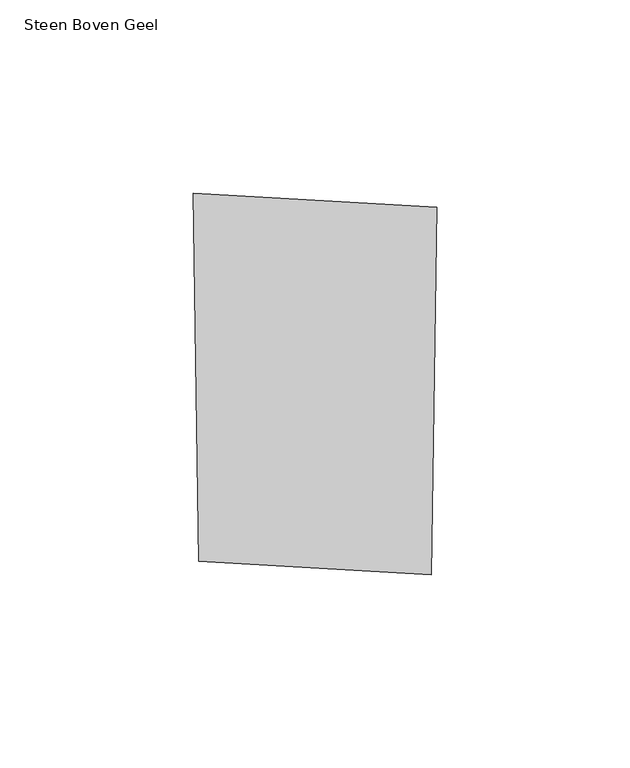
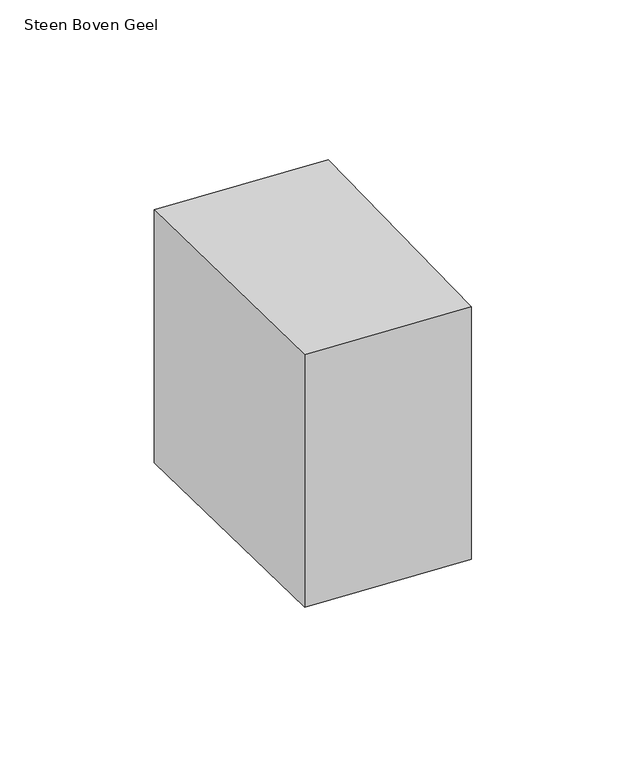
"""IFC4 building model written with IfcOpenShell, lengths in millimetres: proxy geometry, 00_GMA_steen_versie_4 : Steen Boven Geel."""

from ifc_helpers import new_model, si_unit, origin, origin_with_axes, place, context, project, spatial, polyline, outline, extrude, source, transform, mapped, element, save


def steen_boven_geel_85e85a47(model_context):
    return source(origin(), model_context, "Body", "SweptSolid", [
        extrude(outline(polyline([(101.271578, 118.9291664), (99.9224019, 23.8420556), (39.7241554, 27.3305171), (38.3007414, 122.5859361), (101.271578, 118.9291664)])), origin_with_axes(), (0.0, 0.0, 1.0), 100.0),
    ])


if __name__ == "__main__":
    model = new_model("IFC4")
    model_context = context("Model", 3, world=origin())
    ifc_project = project(units=[si_unit("LENGTHUNIT", "METRE", prefix="MILLI")], contexts=[model_context])
    site = spatial("IfcSite", under=ifc_project)
    building = spatial("IfcBuilding", under=site)
    placement = place(None, origin())
    steen_boven_geel_shape = steen_boven_geel_85e85a47(model_context)
    element("IfcBuildingElementProxy", 1, Name="00_GMA_steen_versie_4 : Steen Boven Geel", ObjectType="00_GMA_steen_versie_4 : Steen Boven Geel", at=placement, inside=building, context=model_context, shape_type="MappedRepresentation", body=[
        mapped(steen_boven_geel_shape, transform((0.0, 0.0, 0.0), x_axis=(1.0, 0.0, 0.0), y_axis=(0.0, 1.0, 0.0), z_axis=(0.0, 0.0, 1.0))),
    ])
    save(model, "model.ifc")

# Revit data of these elements
# Type "00_GMA_steen_versie_4 : Steen Boven Geel"
#   StootVoegHalfBoven [instance default] = 5 mm
#   StootVoegHalf [instance default] = 5 mm
#   StootVoegBreedteOnder = 10 mm
#   StootVoegBreedteBoven = 10 mm
#   Steendikte = 100 mm
#   LintVoegOnderHalf = 5 mm
#   LintVoegOnder = 10 mm
#   LintVoegBovenHalf = 0 mm
#   LintVoegBoven = 0 mm
#   materiaal = 21_steen_geel
#   MateriaalVoeg = none
#   Default Elevation = 0
# Element 1 (IfcBuildingElementProxy, "00_GMA_steen_versie_4 : Steen Boven Geel")
#   Materials on its faces: "21_steen_geel"
# Materials
#   "21_steen_geel": class "Unassigned", colour RGB 202 202 0, transparency 0, Cost = 0
